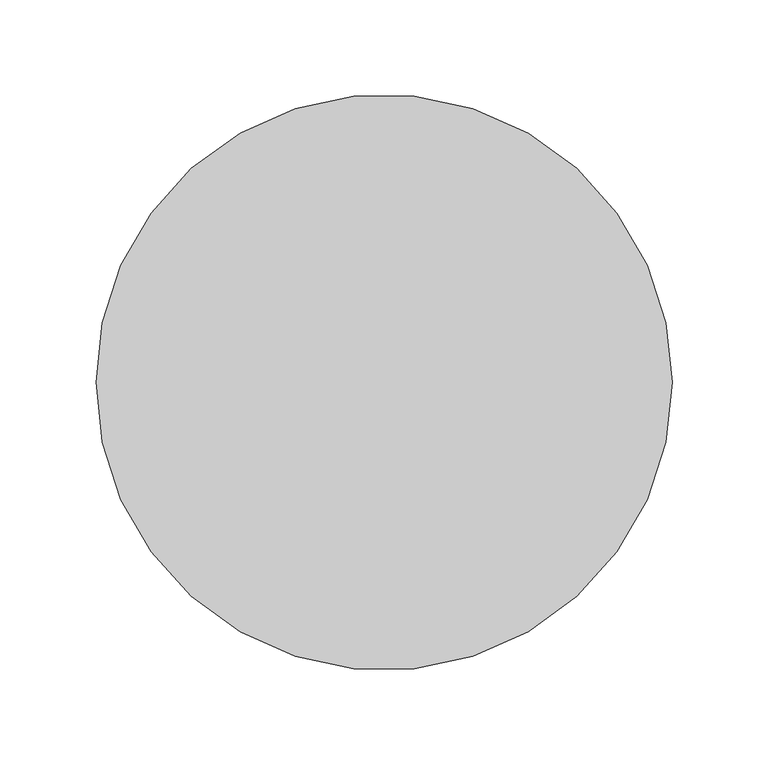
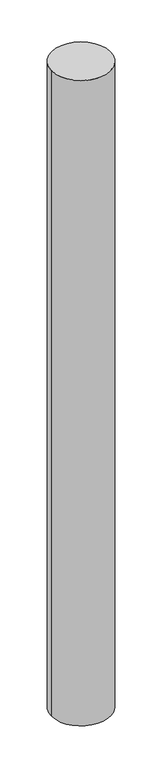
"""IFC4 building model written with IfcOpenShell, lengths in millimetres: column geometry, S-Column_CastInPlace_Round : Ø300."""

from ifc_helpers import new_model, si_unit, point, origin, origin_with_axes, origin_2d, place, context, project, spatial, circle_curve, trimmed, segment, composite_curve, outline, extrude, source, transform, mapped, element, save


def column_bdfed939(model_context):
    return source(origin(), model_context, "Body", "SweptSolid", [
        extrude(outline(composite_curve([segment(trimmed(circle_curve(origin_2d(), 150.0), [point((-150.0, 0.0))], [point((150.0, 0.0))], False, "CARTESIAN"), True, "CONTINUOUS"), segment(trimmed(circle_curve(origin_2d(), 150.0), [point((150.0, 0.0))], [point((-150.0, 0.0))], False, "CARTESIAN"), True, "CONTINUOUS")], self_intersect=False)), origin_with_axes(), (0.0, 0.0, 1.0), 3500.0),
    ])


if __name__ == "__main__":
    model = new_model("IFC4")
    model_context = context("Model", 3, world=origin())
    ifc_project = project(units=[si_unit("LENGTHUNIT", "METRE", prefix="MILLI")], contexts=[model_context])
    site = spatial("IfcSite", under=ifc_project)
    building = spatial("IfcBuilding", under=site)
    placement = place(None, origin())
    column_shape = column_bdfed939(model_context)
    element("IfcColumn", 1, ObjectType="S-Column_CastInPlace_Round : Ø300", at=placement, inside=building, context=model_context, shape_type="MappedRepresentation", body=[
        mapped(column_shape, transform((0.0, 0.0, 0.0), x_axis=(1.0, 0.0, 0.0), y_axis=(0.0, 1.0, 0.0), z_axis=(0.0, 0.0, 1.0))),
    ])
    save(model, "model.ifc")

# Revit data of these elements
# Type "S-Column_CastInPlace_Round : Ø300"
#   NS3457-8 Code = "ASA"
#   NS3451 Code = "2220"
#   NS3457-8 = "ASA Konstruktive søyler"
#   NS3451 = "2220 Søyler"
#   Manufacturer = "Norconsult"
#   Description = "Plasstøpt"
#   Diameter = 300 mm
#   Structural Material = Concrete - Cast In Place
#   Assembly Code = ""
# Element 1 (IfcColumn, "S-Column_CastInPlace_Round : Ø300")
#   Materials on its faces: "Concrete - Cast In Place"
# Materials
#   "Concrete - Cast In Place": class "Concrete", colour RGB 186 186 186, transparency 0, Cost = 0
